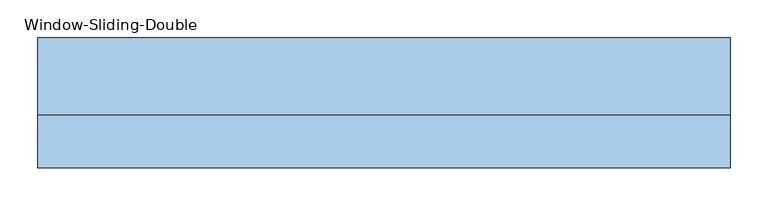
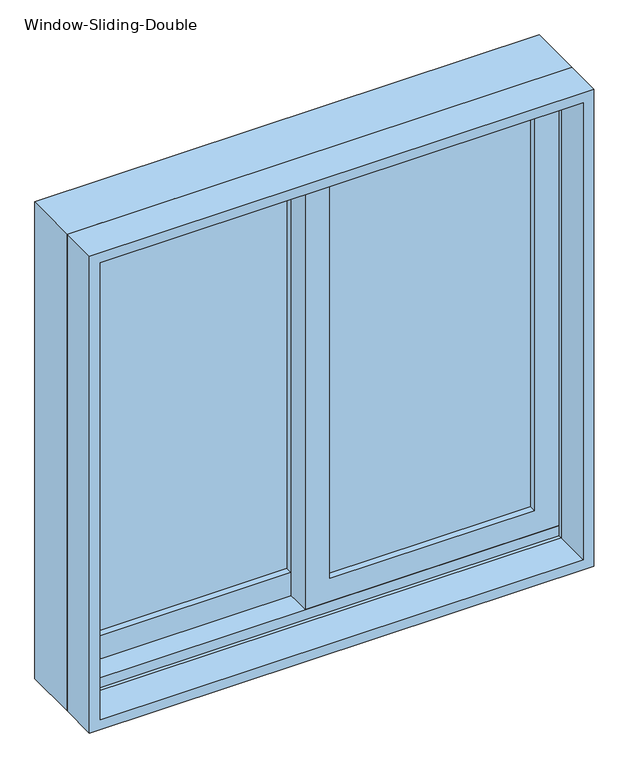
"""IFC4 building model written with IfcOpenShell, lengths in millimetres: window geometry, Window-Sliding-Double."""

from ifc_helpers import new_model, si_unit, frame, origin, place, context, project, spatial, polyline, outline, extrude, faceted_brep, source, transform, mapped, element, save


def window_sliding_double_f2af1e65(model_context):
    return source(origin(), model_context, "Body", "SolidModel", [
        faceted_brep([(-457.2, -10.16, 914.4), (-457.2, 91.44, 914.4), (457.2, 91.44, 914.4), (457.2, -10.16, 914.4), (-416.2778905, 91.44, 1787.8778905), (-416.2778905, 85.09, 1787.8778905), (-416.2778905, 85.09, 933.45), (-416.2778905, 91.44, 933.45), (416.2778905, 85.09, 1787.8778905), (416.2778905, 85.09, 933.45), (438.15, 85.09, 933.45), (438.15, 85.09, 1809.75), (-438.15, 85.09, 1809.75), (-438.15, 85.09, 933.45), (-438.15, -10.16, 1809.75), (-438.15, -10.16, 933.45), (-438.15, -3.81, 933.45), (-438.15, -3.81, 952.5), (-438.15, 40.64, 952.5), (-438.15, 40.64, 933.45), (457.2, -10.16, 1828.8), (-457.2, -10.16, 1828.8), (438.15, -10.16, 1809.75), (438.15, -10.16, 933.45), (-457.2, 91.44, 1828.8), (457.2, 91.44, 1828.8), (416.2778905, 91.44, 933.45), (416.2778905, 91.44, 1787.8778905), (438.15, 40.64, 933.45), (438.15, 40.64, 952.5), (438.15, -3.81, 952.5), (438.15, -3.81, 933.45)], [[[0, 1, 2, 3]], [[4, 5, 6, 7]], [[5, 8, 9, 10, 11, 12, 13, 6]], [[12, 14, 15, 16, 17, 18, 19, 13]], [[0, 3, 20, 21], [22, 23, 15, 14]], [[24, 1, 0, 21]], [[2, 1, 24, 25], [4, 7, 26, 27]], [[5, 4, 27, 8]], [[12, 11, 22, 14]], [[21, 20, 25, 24]], [[8, 27, 26, 9]], [[22, 11, 10, 28, 29, 30, 31, 23]], [[20, 3, 2, 25]], [[26, 7, 6, 13, 19, 28, 10, 9]], [[28, 19, 18, 29]], [[29, 18, 17, 30]], [[30, 17, 16, 31]], [[15, 23, 31, 16]]]),
        extrude(outline(polyline([(1828.8, -457.2), (914.4, -457.2), (914.4, 457.2), (1828.8, 457.2), (1828.8, -457.2)]), holes=[polyline([(1809.75, 438.15), (933.45, 438.15), (933.45, -438.15), (1809.75, -438.15), (1809.75, 438.15)])]), frame((0.0, -80.01, 0.0), z_axis=(0.0, 1.0, 0.0), x_axis=(0.0, 0.0, 1.0)), (0.0, 0.0, 1.0), 69.85),
        extrude(outline(polyline([(393.7, 27.94), (393.7, 21.59), (22.225, 21.59), (22.225, 27.94), (393.7, 27.94)])), frame((0.0, 0.0, 996.95), z_axis=(0.0, 0.0, 1.0), x_axis=(1.0, 0.0, 0.0)), (0.0, 0.0, 1.0), 768.35),
        extrude(outline(polyline([(393.7, 15.24), (393.7, 8.89), (22.225, 8.89), (22.225, 15.24), (393.7, 15.24)])), frame((0.0, 0.0, 996.95), z_axis=(0.0, 0.0, 1.0), x_axis=(1.0, 0.0, 0.0)), (0.0, 0.0, 1.0), 768.35),
        extrude(outline(polyline([(-22.225, 72.39), (-22.225, 66.04), (-393.7, 66.04), (-393.7, 72.39), (-22.225, 72.39)])), frame((0.0, 0.0, 996.95), z_axis=(0.0, 0.0, 1.0), x_axis=(1.0, 0.0, 0.0)), (0.0, 0.0, 1.0), 768.35),
        extrude(outline(polyline([(-22.225, 59.69), (-22.225, 53.34), (-393.7, 53.34), (-393.7, 59.69), (-22.225, 59.69)])), frame((0.0, 0.0, 996.95), z_axis=(0.0, 0.0, 1.0), x_axis=(1.0, 0.0, 0.0)), (0.0, 0.0, 1.0), 768.35),
        extrude(outline(polyline([(933.45, -438.15), (933.45, 22.225), (1809.75, 22.225), (1809.75, -438.15), (933.45, -438.15)]), holes=[polyline([(1765.3, -22.225), (996.95, -22.225), (996.95, -393.7), (1765.3, -393.7), (1765.3, -22.225)])]), frame((0.0, 40.64, 0.0), z_axis=(0.0, 1.0, 0.0), x_axis=(0.0, 0.0, 1.0)), (0.0, 0.0, 1.0), 44.45),
        extrude(outline(polyline([(952.5, 438.15), (1809.75, 438.15), (1809.75, -22.225), (952.5, -22.225), (952.5, 438.15)]), holes=[polyline([(996.95, 22.225), (1765.3, 22.225), (1765.3, 393.7), (996.95, 393.7), (996.95, 22.225)])]), frame((0.0, -3.81, 0.0), z_axis=(0.0, 1.0, 0.0), x_axis=(0.0, 0.0, 1.0)), (0.0, 0.0, 1.0), 44.45),
    ])


if __name__ == "__main__":
    model = new_model("IFC4")
    model_context = context("Model", 3, world=origin())
    ifc_project = project(units=[si_unit("LENGTHUNIT", "METRE", prefix="MILLI")], contexts=[model_context])
    site = spatial("IfcSite", under=ifc_project)
    building = spatial("IfcBuilding", under=site)
    placement = place(None, origin())
    window_sliding_double_shape = window_sliding_double_f2af1e65(model_context)
    element("IfcWindow", 1, ObjectType="Window-Sliding-Double : 3' 10 1/2\" x 2'' 10 1/4\"", at=placement, inside=building, context=model_context, shape_type="MappedRepresentation", body=[
        mapped(window_sliding_double_shape, transform((0.0, 0.0, 0.0), x_axis=(1.0, 0.0, 0.0), y_axis=(0.0, 1.0, 0.0), z_axis=(0.0, 0.0, 1.0))),
    ])
    save(model, "model.ifc")

# Revit data of these elements
# Type "Window-Sliding-Double : 3' 10 1/2\" x 2'' 10 1/4\""
#   Type Mark = "22"
#   Fire Rating = "0.5h"
#   Assembly Code = "B2020100"
#   Analytic Construction = "Double glazing - domestic"
#   Window Inset [instance default] = 0' - 0"
#   Wall Thickness [instance default] = 0' - 6"
#   Visual Light Transmittance = 0.81
#   Thermal Resistance (R) = 0.319569 (m²·K)/W
#   Solar Heat Gain Coefficient = 0.76
#   Muntin Width = 1' - 2 5/8"
#   Muntin Height = 2' - 6 1/4"
#   Interior Wall Closure [instance default] = 0' - 2 3/4"
#   Heat Transfer Coefficient (U) = 3.12929 W/(m²·K)
#   Frame Extension [instance default] = 0' - 0 1/4"
#   Exterior Wall Closure [instance default] = 0' - 1 1/4"
#   Rough Width = 3' - 0 1/2"
#   Rough Height = 3' - 0 1/2"
#   Height = 3' - 0"
#   Extension Jamb [instance default] = 0' - 2 3/4"
#   Default Sill Height = 3' - 0"
#   Width = 3' - 0"
#   Interior Trim Visibility [instance default] = yes
#   Indicator Visibility [instance default] = yes
#   Exterior Trim Visibility [instance default] = yes
#   Muntin Visibility = no
#   Extension Jamb Visibility [instance default] = yes
#   Muntin Pattern = Muntin Pattern_2x2 : Muntin Pattern_2x2
#   Interior Trim Material = Wood - Stained
#   Interior Trim = Trim-Window-Interior-Flat : Picture Frame
#   Interior Frame Material = Wood - Stained
#   Glass Panel Material = Glass
#   Exterior Trim Material = Clad - White
#   Exterior Trim = Trim-Window-Exterior-Flat : with Sill
#   Exterior Frame Material = Clad - White
#   Wall Closure = (empty or 0)
# Element 1 (IfcWindow, "Window-Sliding-Double : 3' 10 1/2\" x 2'' 10 1/4\"")
#   Materials on its faces: "Wood - Stained", "Glass", "Clad - White"
# Materials
#   "Wood - Stained": class "Wood", colour RGB 224 178 126, transparency 0, Cost = 0
#   "Glass": class "Glass", colour RGB 218 227 224, transparency 0.85, Description = "Soda Lime Glass", Cost = 0
#   "Clad - White": class "Wood", colour RGB 242 242 238, transparency 0, Cost = 0
